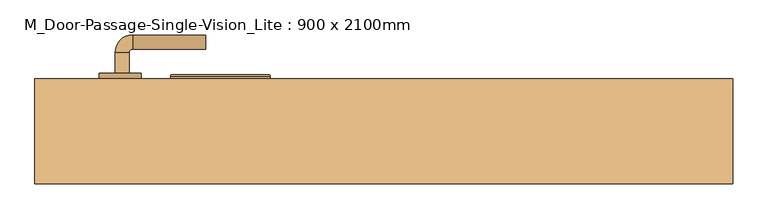
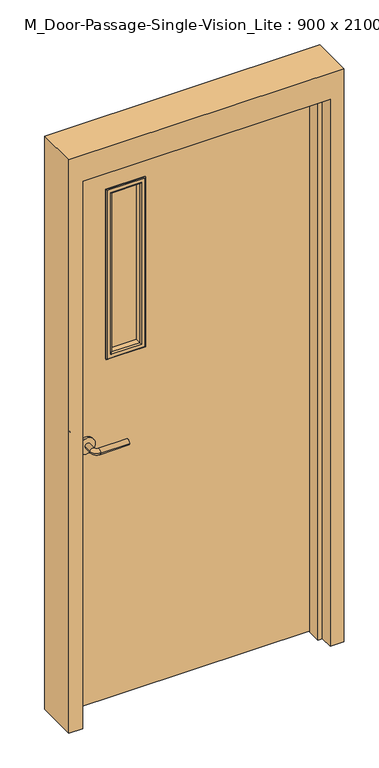
"""IFC4 building model written with IfcOpenShell, lengths in millimetres: door geometry, M_Door-Passage-Single-Vision_Lite : 900 x 2100mm."""

from ifc_helpers import new_model, si_unit, point, frame, frame_2d, origin, place, context, project, spatial, polyline, circle_curve, ellipse_curve, trimmed, segment, composite_curve, outline, extrude, faceted_brep, source, transform, mapped, element, save
from ifc_brep_helpers import plane_surface, cylinder_surface, revolved_surface, advanced_brep


def m_door_passage_single_vision_lite_900_x_2100mm_a921e558(model_context):
    return source(origin(), model_context, "Body", "SolidModel", [
        advanced_brep(
        [(-384.990625, -9.15, 1000.0), (-364.990625, -9.15, 1000.0), (-364.990625, -39.15, 1000.0), (-384.990625, -39.15, 1000.0), (-359.990625, -44.15, 1000.0), (-359.990625, -64.15, 1000.0), (-254.990625, -64.15, 1000.0), (-254.990625, -44.15, 1000.0)],
        [
            (0, 1, circle_curve(frame((-374.990625, -9.15, 1000.0), z_axis=(0.0, 1.0, 0.0), x_axis=(1.0, 0.0, 0.0)), 10.0)),
            (1, 0, circle_curve(frame((-374.990625, -9.15, 1000.0), z_axis=(0.0, 1.0, 0.0), x_axis=(1.0, 0.0, 0.0)), 10.0)),
            (1, 2),
            (2, 3, circle_curve(frame((-374.990625, -39.15, 1000.0), z_axis=(0.0, 1.0, 0.0), x_axis=(1.0, 0.0, 0.0)), 10.0)),
            (3, 0),
            (3, 2, circle_curve(frame((-374.990625, -39.15, 1000.0), z_axis=(0.0, 1.0, 0.0), x_axis=(1.0, 0.0, 0.0)), 10.0)),
            (4, 5, circle_curve(frame((-359.990625, -54.15, 1000.0), z_axis=(-1.0, 0.0, 0.0), x_axis=(0.0, 1.0, 0.0)), 10.0)),
            (5, 3, circle_curve(frame((-359.990625, -39.15, 1000.0), z_axis=(0.0, 0.0, -1.0), x_axis=(-1.0, 0.0, 0.0)), 25.0)),
            (2, 4, circle_curve(frame((-359.990625, -39.15, 1000.0), z_axis=(0.0, 0.0, 1.0), x_axis=(-1.0, 0.0, 0.0)), 5.0)),
            (5, 4, circle_curve(frame((-359.990625, -54.15, 1000.0), z_axis=(-1.0, 0.0, 0.0), x_axis=(0.0, 1.0, 0.0)), 10.0)),
            (6, 7, circle_curve(frame((-254.990625, -54.15, 1000.0), z_axis=(1.0, 0.0, 0.0), x_axis=(0.0, 1.0, 0.0)), 10.0)),
            (7, 6, circle_curve(frame((-254.990625, -54.15, 1000.0), z_axis=(1.0, 0.0, 0.0), x_axis=(0.0, 1.0, 0.0)), 10.0)),
            (4, 7),
            (6, 5),
        ],
        [
            plane_surface(frame((-374.990625, -9.15, 1000.0), z_axis=(0.0, 1.0, 0.0), x_axis=(0.0, 0.0, 1.0))),
            cylinder_surface(frame((-374.990625, -9.15, 1000.0), z_axis=(0.0, 1.0, 0.0), x_axis=(1.0, 0.0, 0.0)), 10.0),
            revolved_surface(trimmed(ellipse_curve(frame((-374.990625, -39.15, 1000.0), z_axis=(0.0, -1.0, 0.0), x_axis=(1.0, 0.0, 0.0)), 10.0, 10.0), [point((-384.990625, -39.15, 1000.0))], [point((-364.990625, -39.15, 1000.0))], True, "CARTESIAN"), (-359.990625, -39.15, 1000.0), (0.0, 0.0, -1.0)),
            revolved_surface(trimmed(ellipse_curve(frame((-374.990625, -39.15, 1000.0), z_axis=(0.0, -1.0, 0.0), x_axis=(1.0, 0.0, 0.0)), 10.0, 10.0), [point((-364.990625, -39.15, 1000.0))], [point((-384.990625, -39.15, 1000.0))], True, "CARTESIAN"), (-359.990625, -39.15, 1000.0), (0.0, 0.0, -1.0)),
            plane_surface(frame((-254.990625, -54.15, 1000.0), z_axis=(1.0, 0.0, 0.0), x_axis=(0.0, 0.0, 1.0))),
            cylinder_surface(frame((-359.990625, -54.15, 1000.0), z_axis=(-1.0, 0.0, 0.0), x_axis=(0.0, 1.0, 0.0)), 10.0),
        ],
        [
            (0, [[1, 2]]),
            (1, [[3, 4, 5, -2]]),
            (1, [[-5, 6, -3, -1]]),
            (2, [[7, 8, -4, 9]]),
            (3, [[10, -9, -6, -8]]),
            (4, [[11, 12]]),
            (5, [[13, -11, 14, -7]]),
            (5, [[-14, -12, -13, -10]]),
        ],
    ),
        extrude(outline(composite_curve([segment(trimmed(circle_curve(frame_2d((1000.0, -377.490625)), 30.0), [point((1000.0, -407.490625))], [point((1000.0, -347.490625))], False, "CARTESIAN"), True, "CONTINUOUS"), segment(trimmed(circle_curve(frame_2d((1000.0, -377.490625)), 30.0), [point((1000.0, -347.490625))], [point((1000.0, -407.490625))], False, "CARTESIAN"), True, "CONTINUOUS")], self_intersect=False)), frame((0.0, -9.15, 0.0), z_axis=(0.0, 1.0, 0.0), x_axis=(0.0, 0.0, 1.0)), (0.0, 0.0, 1.0), 8.0),
        advanced_brep(
        [(-384.990625, 51.85, 1000.0), (-364.990625, 51.85, 1000.0), (-384.990625, 81.85, 1000.0), (-364.990625, 81.85, 1000.0), (-359.990625, 86.85, 1000.0), (-359.990625, 106.85, 1000.0), (-254.990625, 106.85, 1000.0), (-254.990625, 86.85, 1000.0)],
        [
            (0, 1, circle_curve(frame((-374.990625, 51.85, 1000.0), z_axis=(0.0, -1.0, 0.0), x_axis=(1.0, 0.0, 0.0)), 10.0)),
            (1, 0, circle_curve(frame((-374.990625, 51.85, 1000.0), z_axis=(0.0, -1.0, 0.0), x_axis=(1.0, 0.0, 0.0)), 10.0)),
            (0, 2),
            (2, 3, circle_curve(frame((-374.990625, 81.85, 1000.0), z_axis=(0.0, -1.0, 0.0), x_axis=(1.0, 0.0, 0.0)), 10.0)),
            (3, 1),
            (3, 2, circle_curve(frame((-374.990625, 81.85, 1000.0), z_axis=(0.0, -1.0, 0.0), x_axis=(1.0, 0.0, 0.0)), 10.0)),
            (4, 3, circle_curve(frame((-359.990625, 81.85, 1000.0), z_axis=(0.0, 0.0, 1.0), x_axis=(-1.0, 0.0, 0.0)), 5.0)),
            (2, 5, circle_curve(frame((-359.990625, 81.85, 1000.0), z_axis=(0.0, 0.0, -1.0), x_axis=(-1.0, 0.0, 0.0)), 25.0)),
            (5, 4, circle_curve(frame((-359.990625, 96.85, 1000.0), z_axis=(-1.0, 0.0, 0.0), x_axis=(0.0, -1.0, 0.0)), 10.0)),
            (4, 5, circle_curve(frame((-359.990625, 96.85, 1000.0), z_axis=(-1.0, 0.0, 0.0), x_axis=(0.0, -1.0, 0.0)), 10.0)),
            (6, 7, circle_curve(frame((-254.990625, 96.85, 1000.0), z_axis=(1.0, 0.0, 0.0), x_axis=(0.0, -1.0, 0.0)), 10.0)),
            (7, 6, circle_curve(frame((-254.990625, 96.85, 1000.0), z_axis=(1.0, 0.0, 0.0), x_axis=(0.0, -1.0, 0.0)), 10.0)),
            (5, 6),
            (7, 4),
        ],
        [
            plane_surface(frame((-374.990625, 51.85, 1000.0), z_axis=(0.0, -1.0, 0.0), x_axis=(0.0, 0.0, 1.0))),
            cylinder_surface(frame((-374.990625, 51.85, 1000.0), z_axis=(0.0, -1.0, 0.0), x_axis=(1.0, 0.0, 0.0)), 10.0),
            revolved_surface(trimmed(ellipse_curve(frame((-374.990625, 81.85, 1000.0), z_axis=(0.0, -1.0, 0.0), x_axis=(1.0, 0.0, 0.0)), 10.0, 10.0), [point((-384.990625, 81.85, 1000.0))], [point((-364.990625, 81.85, 1000.0))], True, "CARTESIAN"), (-359.990625, 81.85, 1000.0), (0.0, 0.0, -1.0)),
            revolved_surface(trimmed(ellipse_curve(frame((-374.990625, 81.85, 1000.0), z_axis=(0.0, -1.0, 0.0), x_axis=(1.0, 0.0, 0.0)), 10.0, 10.0), [point((-364.990625, 81.85, 1000.0))], [point((-384.990625, 81.85, 1000.0))], True, "CARTESIAN"), (-359.990625, 81.85, 1000.0), (0.0, 0.0, -1.0)),
            plane_surface(frame((-254.990625, 96.85, 1000.0), z_axis=(1.0, 0.0, 0.0), x_axis=(0.0, 0.0, 1.0))),
            cylinder_surface(frame((-359.990625, 96.85, 1000.0), z_axis=(-1.0, 0.0, 0.0), x_axis=(0.0, -1.0, 0.0)), 10.0),
        ],
        [
            (0, [[1, 2]]),
            (1, [[-1, 3, 4, 5]]),
            (1, [[-2, -5, 6, -3]]),
            (2, [[7, -4, 8, 9]]),
            (3, [[-8, -6, -7, 10]]),
            (4, [[11, 12]]),
            (5, [[-9, 13, -12, 14]]),
            (5, [[-10, -14, -11, -13]]),
        ],
    ),
        extrude(outline(composite_curve([segment(trimmed(circle_curve(frame_2d((1000.0, -377.490625)), 30.0), [point((1000.0, -407.490625))], [point((1000.0, -347.490625))], False, "CARTESIAN"), True, "CONTINUOUS"), segment(trimmed(circle_curve(frame_2d((1000.0, -377.490625)), 30.0), [point((1000.0, -347.490625))], [point((1000.0, -407.490625))], False, "CARTESIAN"), True, "CONTINUOUS")], self_intersect=False)), frame((0.0, 43.85, 0.0), z_axis=(0.0, 1.0, 0.0), x_axis=(0.0, 0.0, 1.0)), (0.0, 0.0, 1.0), 8.0),
        extrude(outline(polyline([(2100.0, -450.0), (0.0, -450.0), (0.0, 450.0), (2100.0, 450.0), (2100.0, -450.0)]), holes=[polyline([(1947.6, -297.6), (1947.6, -170.6), (1312.6, -170.6), (1312.6, -297.6), (1947.6, -297.6)])]), frame((0.0, -1.15, 0.0), z_axis=(0.0, 1.0, 0.0), x_axis=(0.0, 0.0, 1.0)), (0.0, 0.0, 1.0), 45.0),
        faceted_brep([(450.0, -5.9125, 0.0), (450.0, 43.85, 0.0), (500.0, 43.85, 0.0), (500.0, -106.15, 0.0), (450.0, -106.15, 0.0), (450.0, -56.9375, 0.0), (434.125, -56.9375, 0.0), (434.125, -5.9125, 0.0), (450.0, -5.9125, 2100.0), (450.0, 43.85, 2100.0), (-450.0, 43.85, 2100.0), (-450.0, 43.85, 0.0), (-500.0, 43.85, 0.0), (-500.0, 43.85, 2200.0), (500.0, 43.85, 2200.0), (500.0, -106.15, 2200.0), (-500.0, -106.15, 2200.0), (-500.0, -106.15, 0.0), (-450.0, -106.15, 0.0), (-450.0, -106.15, 2100.0), (450.0, -106.15, 2100.0), (450.0, -56.9375, 2100.0), (-450.0, -56.9375, 2100.0), (-450.0, -56.9375, 0.0), (-434.125, -56.9375, 0.0), (-434.125, -56.9375, 2084.125), (434.125, -56.9375, 2084.125), (434.125, -5.9125, 2084.125), (-434.125, -5.9125, 2084.125), (-434.125, -5.9125, 0.0), (-450.0, -5.9125, 0.0), (-450.0, -5.9125, 2100.0)], [[[0, 1, 2, 3, 4, 5, 6, 7]], [[1, 0, 8, 9]], [[2, 1, 9, 10, 11, 12, 13, 14]], [[3, 2, 14, 15]], [[4, 3, 15, 16, 17, 18, 19, 20]], [[5, 4, 20, 21]], [[6, 5, 21, 22, 23, 24, 25, 26]], [[7, 6, 26, 27]], [[0, 7, 27, 28, 29, 30, 31, 8]], [[9, 8, 31, 10]], [[20, 19, 22, 21]], [[26, 25, 28, 27]], [[12, 11, 30, 29, 24, 23, 18, 17]], [[11, 10, 31, 30]], [[13, 12, 17, 16]], [[19, 18, 23, 22]], [[25, 24, 29, 28]], [[15, 14, 13, 16]]]),
        extrude(outline(polyline([(-170.6, 18.85), (-297.6, 18.85), (-297.6, 23.85), (-170.6, 23.85), (-170.6, 18.85)])), frame((0.0, 0.0, 1312.6), z_axis=(0.0, 0.0, 1.0), x_axis=(1.0, 0.0, 0.0)), (0.0, 0.0, 1.0), 635.0),
        advanced_brep(
        [(-297.6, 23.85, 1947.6), (-297.6, 43.85, 1947.6), (-297.6, 43.85, 1312.6), (-297.6, 23.85, 1312.6), (-285.6, 44.85, 1935.6), (-285.6, 23.85, 1935.6), (-285.6, 23.85, 1324.6), (-285.6, 44.85, 1324.6), (-290.6, 49.85, 1940.6), (-290.6, 49.85, 1319.6), (-305.6, 47.85, 1955.6), (-303.6, 49.85, 1953.6), (-303.6, 49.85, 1306.6), (-305.6, 47.85, 1304.6), (-305.6, 43.85, 1955.6), (-305.6, 43.85, 1304.6), (-170.6, 43.85, 1312.6), (-170.6, 23.85, 1312.6), (-182.6, 23.85, 1324.6), (-182.6, 44.85, 1324.6), (-177.6, 49.85, 1319.6), (-164.6, 49.85, 1306.6), (-162.6, 47.85, 1304.6), (-162.6, 43.85, 1304.6), (-170.6, 43.85, 1947.6), (-170.6, 23.85, 1947.6), (-182.6, 23.85, 1935.6), (-182.6, 44.85, 1935.6), (-177.6, 49.85, 1940.6), (-164.6, 49.85, 1953.6), (-162.6, 47.85, 1955.6), (-162.6, 43.85, 1955.6)],
        [
            (0, 1),
            (1, 2),
            (2, 3),
            (3, 0),
            (4, 5),
            (5, 6),
            (6, 7),
            (7, 4),
            (8, 4, ellipse_curve(frame((-290.6, 44.85, 1940.6), z_axis=(-0.7071067811865475, 0.0, -0.7071067811865475), x_axis=(-0.7071067811865474, 0.0, 0.7071067811865476)), 7.0710678, 5.0)),
            (7, 9, ellipse_curve(frame((-290.6, 44.85, 1319.6), z_axis=(-0.7071067811865475, 0.0, 0.7071067811865475), x_axis=(0.7071067811865474, 0.0, 0.7071067811865476)), 7.0710678, 5.0)),
            (9, 8),
            (10, 11, ellipse_curve(frame((-303.6, 47.85, 1953.6), z_axis=(-0.7071067811865475, 0.0, -0.7071067811865475), x_axis=(-0.7071067811865474, 0.0, 0.7071067811865476)), 2.8284271, 2.0)),
            (11, 12),
            (12, 13, ellipse_curve(frame((-303.6, 47.85, 1306.6), z_axis=(-0.7071067811865475, 0.0, 0.7071067811865475), x_axis=(0.7071067811865474, 0.0, 0.7071067811865476)), 2.8284271, 2.0)),
            (13, 10),
            (14, 10),
            (13, 15),
            (15, 14),
            (2, 16),
            (16, 17),
            (17, 3),
            (6, 18),
            (18, 19),
            (19, 7),
            (19, 20, ellipse_curve(frame((-177.6, 44.85, 1319.6), z_axis=(-0.7071067811865475, 0.0, -0.7071067811865475), x_axis=(-0.7071067811865476, 0.0, 0.7071067811865474)), 7.0710678, 5.0)),
            (20, 9),
            (12, 21),
            (21, 22, ellipse_curve(frame((-164.6, 47.85, 1306.6), z_axis=(-0.7071067811865475, 0.0, -0.7071067811865475), x_axis=(-0.7071067811865476, 0.0, 0.7071067811865474)), 2.8284271, 2.0)),
            (22, 13),
            (22, 23),
            (23, 15),
            (16, 24),
            (24, 25),
            (25, 17),
            (18, 26),
            (26, 27),
            (27, 19),
            (27, 28, ellipse_curve(frame((-177.6, 44.85, 1940.6), z_axis=(0.7071067811865475, 0.0, -0.7071067811865475), x_axis=(-0.7071067811865474, 0.0, -0.7071067811865476)), 7.0710678, 5.0)),
            (28, 20),
            (21, 29),
            (29, 30, ellipse_curve(frame((-164.6, 47.85, 1953.6), z_axis=(0.7071067811865475, 0.0, -0.7071067811865475), x_axis=(-0.7071067811865474, 0.0, -0.7071067811865476)), 2.8284271, 2.0)),
            (30, 22),
            (30, 31),
            (31, 23),
            (31, 14),
            (1, 24),
            (0, 25),
            (5, 26),
            (4, 27),
            (8, 28),
            (11, 29),
            (10, 30),
        ],
        [
            plane_surface(frame((-297.6, 43.85, 1947.6), z_axis=(-1.0, 0.0, 0.0), x_axis=(0.0, 0.0, -1.0))),
            plane_surface(frame((-285.6, 23.85, 1935.6), z_axis=(1.0, 0.0, 0.0), x_axis=(0.0, 0.0, -1.0))),
            cylinder_surface(frame((-290.6, 44.85, 1947.6), z_axis=(0.0, 0.0, 1.0), x_axis=(-1.0, 0.0, 0.0)), 5.0),
            cylinder_surface(frame((-303.6, 47.85, 1947.6), z_axis=(0.0, 0.0, 1.0), x_axis=(-1.0, 0.0, 0.0)), 2.0),
            plane_surface(frame((-305.6, 47.85, 1955.6), z_axis=(-1.0, 0.0, 0.0), x_axis=(0.0, 0.0, -1.0))),
            plane_surface(frame((-297.6, 43.85, 1312.6), z_axis=(0.0, 0.0, -1.0), x_axis=(1.0, 0.0, 0.0))),
            plane_surface(frame((-285.6, 23.85, 1324.6), z_axis=(0.0, 0.0, 1.0), x_axis=(1.0, 0.0, 0.0))),
            cylinder_surface(frame((-297.6, 44.85, 1319.6), z_axis=(-1.0, 0.0, 0.0), x_axis=(0.0, 0.0, -1.0)), 5.0),
            cylinder_surface(frame((-297.6, 47.85, 1306.6), z_axis=(-1.0, 0.0, 0.0), x_axis=(0.0, 0.0, -1.0)), 2.0),
            plane_surface(frame((-305.6, 47.85, 1304.6), z_axis=(0.0, 0.0, -1.0), x_axis=(1.0, 0.0, 0.0))),
            plane_surface(frame((-170.6, 43.85, 1312.6), z_axis=(1.0, 0.0, 0.0), x_axis=(0.0, 0.0, 1.0))),
            plane_surface(frame((-182.6, 23.85, 1324.6), z_axis=(-1.0, 0.0, 0.0), x_axis=(0.0, 0.0, 1.0))),
            cylinder_surface(frame((-177.6, 44.85, 1312.6), z_axis=(0.0, 0.0, -1.0), x_axis=(1.0, 0.0, 0.0)), 5.0),
            cylinder_surface(frame((-164.6, 47.85, 1312.6), z_axis=(0.0, 0.0, -1.0), x_axis=(1.0, 0.0, 0.0)), 2.0),
            plane_surface(frame((-162.6, 47.85, 1304.6), z_axis=(1.0, 0.0, 0.0), x_axis=(0.0, 0.0, 1.0))),
            plane_surface(frame((-162.6, 43.85, 1955.6), z_axis=(0.0, -1.0, 0.0), x_axis=(-1.0, 0.0, 0.0))),
            plane_surface(frame((-170.6, 43.85, 1947.6), z_axis=(0.0, 0.0, 1.0), x_axis=(-1.0, 0.0, 0.0))),
            plane_surface(frame((-170.6, 23.85, 1947.6), z_axis=(0.0, -1.0, 0.0), x_axis=(-1.0, 0.0, 0.0))),
            plane_surface(frame((-182.6, 23.85, 1935.6), z_axis=(0.0, 0.0, -1.0), x_axis=(-1.0, 0.0, 0.0))),
            cylinder_surface(frame((-170.6, 44.85, 1940.6), z_axis=(1.0, 0.0, 0.0), x_axis=(0.0, 0.0, 1.0)), 5.0),
            plane_surface(frame((-177.6, 49.85, 1940.6), z_axis=(0.0, 1.0, 0.0), x_axis=(-1.0, 0.0, 0.0))),
            cylinder_surface(frame((-170.6, 47.85, 1953.6), z_axis=(1.0, 0.0, 0.0), x_axis=(0.0, 0.0, 1.0)), 2.0),
            plane_surface(frame((-162.6, 47.85, 1955.6), z_axis=(0.0, 0.0, 1.0), x_axis=(-1.0, 0.0, 0.0))),
        ],
        [
            (0, [[1, 2, 3, 4]]),
            (1, [[5, 6, 7, 8]]),
            (2, [[9, -8, 10, 11]]),
            (3, [[12, 13, 14, 15]]),
            (4, [[16, -15, 17, 18]]),
            (5, [[-3, 19, 20, 21]]),
            (6, [[-7, 22, 23, 24]]),
            (7, [[-10, -24, 25, 26]]),
            (8, [[-14, 27, 28, 29]]),
            (9, [[-17, -29, 30, 31]]),
            (10, [[-20, 32, 33, 34]]),
            (11, [[-23, 35, 36, 37]]),
            (12, [[-25, -37, 38, 39]]),
            (13, [[-28, 40, 41, 42]]),
            (14, [[-30, -42, 43, 44]]),
            (15, [[-31, -44, 45, -18], [46, -32, -19, -2]]),
            (16, [[-33, -46, -1, 47]]),
            (17, [[-21, -34, -47, -4], [48, -35, -22, -6]]),
            (18, [[-36, -48, -5, 49]]),
            (19, [[-38, -49, -9, 50]]),
            (20, [[51, -40, -27, -13], [-26, -39, -50, -11]]),
            (21, [[-41, -51, -12, 52]]),
            (22, [[-43, -52, -16, -45]]),
        ],
    ),
        advanced_brep(
        [(-297.6, 18.85, 1312.6), (-297.6, -1.15, 1312.6), (-297.6, -1.15, 1947.6), (-297.6, 18.85, 1947.6), (-285.6, -2.15, 1324.6), (-285.6, 18.85, 1324.6), (-285.6, 18.85, 1935.6), (-285.6, -2.15, 1935.6), (-290.6, -7.15, 1319.6), (-290.6, -7.15, 1940.6), (-305.6, -5.15, 1304.6), (-303.6, -7.15, 1306.6), (-303.6, -7.15, 1953.6), (-305.6, -5.15, 1955.6), (-305.6, -1.15, 1304.6), (-305.6, -1.15, 1955.6), (-170.6, -1.15, 1947.6), (-170.6, 18.85, 1947.6), (-182.6, 18.85, 1935.6), (-182.6, -2.15, 1935.6), (-177.6, -7.15, 1940.6), (-164.6, -7.15, 1953.6), (-162.6, -5.15, 1955.6), (-162.6, -1.15, 1955.6), (-170.6, -1.15, 1312.6), (-170.6, 18.85, 1312.6), (-182.6, 18.85, 1324.6), (-182.6, -2.15, 1324.6), (-177.6, -7.15, 1319.6), (-164.6, -7.15, 1306.6), (-162.6, -5.15, 1304.6), (-162.6, -1.15, 1304.6)],
        [
            (0, 1),
            (1, 2),
            (2, 3),
            (3, 0),
            (4, 5),
            (5, 6),
            (6, 7),
            (7, 4),
            (8, 4, ellipse_curve(frame((-290.6, -2.15, 1319.6), z_axis=(-0.7071067811865475, 0.0, 0.7071067811865475), x_axis=(-0.7071067811865474, 0.0, -0.7071067811865476)), 7.0710678, 5.0)),
            (7, 9, ellipse_curve(frame((-290.6, -2.15, 1940.6), z_axis=(-0.7071067811865475, 0.0, -0.7071067811865475), x_axis=(0.7071067811865474, 0.0, -0.7071067811865476)), 7.0710678, 5.0)),
            (9, 8),
            (10, 11, ellipse_curve(frame((-303.6, -5.15, 1306.6), z_axis=(-0.7071067811865475, 0.0, 0.7071067811865475), x_axis=(-0.7071067811865474, 0.0, -0.7071067811865476)), 2.8284271, 2.0)),
            (11, 12),
            (12, 13, ellipse_curve(frame((-303.6, -5.15, 1953.6), z_axis=(-0.7071067811865475, 0.0, -0.7071067811865475), x_axis=(0.7071067811865474, 0.0, -0.7071067811865476)), 2.8284271, 2.0)),
            (13, 10),
            (14, 10),
            (13, 15),
            (15, 14),
            (2, 16),
            (16, 17),
            (17, 3),
            (6, 18),
            (18, 19),
            (19, 7),
            (19, 20, ellipse_curve(frame((-177.6, -2.15, 1940.6), z_axis=(-0.7071067811865475, 0.0, 0.7071067811865475), x_axis=(-0.7071067811865476, 0.0, -0.7071067811865474)), 7.0710678, 5.0)),
            (20, 9),
            (12, 21),
            (21, 22, ellipse_curve(frame((-164.6, -5.15, 1953.6), z_axis=(-0.7071067811865475, 0.0, 0.7071067811865475), x_axis=(-0.7071067811865476, 0.0, -0.7071067811865474)), 2.8284271, 2.0)),
            (22, 13),
            (22, 23),
            (23, 15),
            (16, 24),
            (24, 25),
            (25, 17),
            (18, 26),
            (26, 27),
            (27, 19),
            (27, 28, ellipse_curve(frame((-177.6, -2.15, 1319.6), z_axis=(0.7071067811865475, 0.0, 0.7071067811865475), x_axis=(-0.7071067811865474, 0.0, 0.7071067811865476)), 7.0710678, 5.0)),
            (28, 20),
            (21, 29),
            (29, 30, ellipse_curve(frame((-164.6, -5.15, 1306.6), z_axis=(0.7071067811865475, 0.0, 0.7071067811865475), x_axis=(-0.7071067811865474, 0.0, 0.7071067811865476)), 2.8284271, 2.0)),
            (30, 22),
            (30, 31),
            (31, 23),
            (31, 14),
            (1, 24),
            (0, 25),
            (5, 26),
            (4, 27),
            (8, 28),
            (11, 29),
            (10, 30),
        ],
        [
            plane_surface(frame((-297.6, -1.15, 1312.6), z_axis=(-1.0, 0.0, 0.0), x_axis=(0.0, 0.0, 1.0))),
            plane_surface(frame((-285.6, 18.85, 1324.6), z_axis=(1.0, 0.0, 0.0), x_axis=(0.0, 0.0, 1.0))),
            cylinder_surface(frame((-290.6, -2.15, 1312.6), z_axis=(0.0, 0.0, -1.0), x_axis=(-1.0, 0.0, 0.0)), 5.0),
            cylinder_surface(frame((-303.6, -5.15, 1312.6), z_axis=(0.0, 0.0, -1.0), x_axis=(-1.0, 0.0, 0.0)), 2.0),
            plane_surface(frame((-305.6, -5.15, 1304.6), z_axis=(-1.0, 0.0, 0.0), x_axis=(0.0, 0.0, 1.0))),
            plane_surface(frame((-297.6, -1.15, 1947.6), z_axis=(0.0, 0.0, 1.0), x_axis=(1.0, 0.0, 0.0))),
            plane_surface(frame((-285.6, 18.85, 1935.6), z_axis=(0.0, 0.0, -1.0), x_axis=(1.0, 0.0, 0.0))),
            cylinder_surface(frame((-297.6, -2.15, 1940.6), z_axis=(-1.0, 0.0, 0.0), x_axis=(0.0, 0.0, 1.0)), 5.0),
            cylinder_surface(frame((-297.6, -5.15, 1953.6), z_axis=(-1.0, 0.0, 0.0), x_axis=(0.0, 0.0, 1.0)), 2.0),
            plane_surface(frame((-305.6, -5.15, 1955.6), z_axis=(0.0, 0.0, 1.0), x_axis=(1.0, 0.0, 0.0))),
            plane_surface(frame((-170.6, -1.15, 1947.6), z_axis=(1.0, 0.0, 0.0), x_axis=(0.0, 0.0, -1.0))),
            plane_surface(frame((-182.6, 18.85, 1935.6), z_axis=(-1.0, 0.0, 0.0), x_axis=(0.0, 0.0, -1.0))),
            cylinder_surface(frame((-177.6, -2.15, 1947.6), z_axis=(0.0, 0.0, 1.0), x_axis=(1.0, 0.0, 0.0)), 5.0),
            cylinder_surface(frame((-164.6, -5.15, 1947.6), z_axis=(0.0, 0.0, 1.0), x_axis=(1.0, 0.0, 0.0)), 2.0),
            plane_surface(frame((-162.6, -5.15, 1955.6), z_axis=(1.0, 0.0, 0.0), x_axis=(0.0, 0.0, -1.0))),
            plane_surface(frame((-162.6, -1.15, 1304.6), z_axis=(0.0, 1.0, 0.0), x_axis=(-1.0, 0.0, 0.0))),
            plane_surface(frame((-170.6, -1.15, 1312.6), z_axis=(0.0, 0.0, -1.0), x_axis=(-1.0, 0.0, 0.0))),
            plane_surface(frame((-170.6, 18.85, 1312.6), z_axis=(0.0, 1.0, 0.0), x_axis=(-1.0, 0.0, 0.0))),
            plane_surface(frame((-182.6, 18.85, 1324.6), z_axis=(0.0, 0.0, 1.0), x_axis=(-1.0, 0.0, 0.0))),
            cylinder_surface(frame((-170.6, -2.15, 1319.6), z_axis=(1.0, 0.0, 0.0), x_axis=(0.0, 0.0, -1.0)), 5.0),
            plane_surface(frame((-177.6, -7.15, 1319.6), z_axis=(0.0, -1.0, 0.0), x_axis=(-1.0, 0.0, 0.0))),
            cylinder_surface(frame((-170.6, -5.15, 1306.6), z_axis=(1.0, 0.0, 0.0), x_axis=(0.0, 0.0, -1.0)), 2.0),
            plane_surface(frame((-162.6, -5.15, 1304.6), z_axis=(0.0, 0.0, -1.0), x_axis=(-1.0, 0.0, 0.0))),
        ],
        [
            (0, [[1, 2, 3, 4]]),
            (1, [[5, 6, 7, 8]]),
            (2, [[9, -8, 10, 11]]),
            (3, [[12, 13, 14, 15]]),
            (4, [[16, -15, 17, 18]]),
            (5, [[-3, 19, 20, 21]]),
            (6, [[-7, 22, 23, 24]]),
            (7, [[-10, -24, 25, 26]]),
            (8, [[-14, 27, 28, 29]]),
            (9, [[-17, -29, 30, 31]]),
            (10, [[-20, 32, 33, 34]]),
            (11, [[-23, 35, 36, 37]]),
            (12, [[-25, -37, 38, 39]]),
            (13, [[-28, 40, 41, 42]]),
            (14, [[-30, -42, 43, 44]]),
            (15, [[-31, -44, 45, -18], [46, -32, -19, -2]]),
            (16, [[-33, -46, -1, 47]]),
            (17, [[-21, -34, -47, -4], [48, -35, -22, -6]]),
            (18, [[-36, -48, -5, 49]]),
            (19, [[-38, -49, -9, 50]]),
            (20, [[51, -40, -27, -13], [-26, -39, -50, -11]]),
            (21, [[-41, -51, -12, 52]]),
            (22, [[-43, -52, -16, -45]]),
        ],
    ),
    ])


if __name__ == "__main__":
    model = new_model("IFC4")
    model_context = context("Model", 3, world=origin())
    ifc_project = project(units=[si_unit("LENGTHUNIT", "METRE", prefix="MILLI")], contexts=[model_context])
    site = spatial("IfcSite", under=ifc_project)
    building = spatial("IfcBuilding", under=site)
    placement = place(None, origin())
    m_door_passage_single_vision_lite_900_x_2100mm_shape = m_door_passage_single_vision_lite_900_x_2100mm_a921e558(model_context)
    element("IfcDoor", 1, ObjectType="M_Door-Passage-Single-Vision_Lite : 900 x 2100mm", at=placement, inside=building, context=model_context, shape_type="MappedRepresentation", body=[
        mapped(m_door_passage_single_vision_lite_900_x_2100mm_shape, transform((0.0, 0.0, 0.0), x_axis=(1.0, 0.0, 0.0), y_axis=(0.0, 1.0, 0.0), z_axis=(0.0, 0.0, 1.0))),
    ])
    save(model, "model.ifc")

# Revit data of these elements
# Type "M_Door-Passage-Single-Vision_Lite : 900 x 2100mm"
#   Type Mark = "45"
#   Assembly Code = "B2030100"
#   Analytic Construction = "Wooden"
#   Thickness = 45 mm
#   Thermal Resistance (R) = 0.455703 (m²·K)/W
#   Swing Angle [instance default] = 90.00°
#   Strike Height = 1000 mm
#   Rough Width [instance default] = 1000 mm
#   Rough Height [instance default] = 2200 mm
#   MFOpeningHeight [instance default] = 100 mm
#   MFOpeningWidth [instance default] = 100 mm
#   Inset Calculate [instance default] = 105 mm
#   Masonry Inset [instance default] = 25 mm
#   Height = 2100 mm
#   Width = 900 mm
#   Heat Transfer Coefficient (U) = 2.19465 W/(m²·K)
#   Masonry Frame Depth = 150 mm
#   Masonry Frame [instance default] = yes
#   Function = 1
#   Dry Wall Frame [instance default] = no
#   Panel Material = Wood - Birch
#   Glazing = Glass
#   Glass Stop Material = Metal - Paint Finish - Grey
#   Frame Material = Metal - Paint Finish - Grey
#   Door Handle Material = Aluminum
#   Visual Light Transmittance = 0
#   Solar Heat Gain Coefficient = 0
#   Wall Closure = (empty or 0)
# Element 1 (IfcDoor, "M_Door-Passage-Single-Vision_Lite : 900 x 2100mm")
#   Materials on its faces: "Metal - Paint Finish - Grey", "Aluminum", "Wood - Birch", "Glass"
# Materials
#   "Wood - Birch": class "Wood", colour RGB 173 132 96, transparency 0, Cost = 0
#   "Glass": class "Glass", colour RGB 245 245 243, transparency 1, Description = "Soda Lime Glass", Cost = 0
#   "Metal - Paint Finish - Grey": class "Paint", colour RGB 178 178 178, transparency 0, Cost = 0
#   "Aluminum": class "Metal", colour RGB 244 245 246, transparency 0, Description = "Aluminum 6061", Cost = 0
